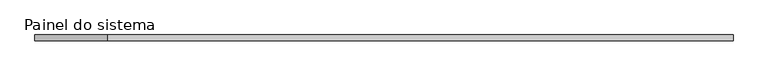
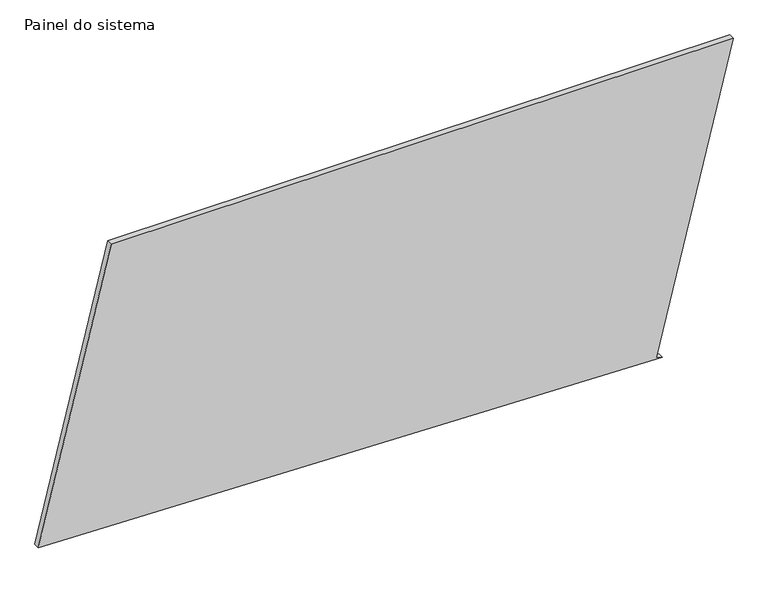
"""IFC4 building model written with IfcOpenShell, lengths in millimetres: plate geometry, Painel do sistema : Envidraçado."""

from ifc_helpers import new_model, si_unit, frame, origin, place, context, project, spatial, polyline, outline, extrude, source, transform, mapped, element, save


def painel_do_sistema_4682d0e1(model_context):
    return source(origin(), model_context, "Body", "SweptSolid", [
        extrude(outline(polyline([(0.0, 1166.435661), (5.9765403, 1142.160551), (1318.2584981, 1465.2448107), (1318.2584981, -1158.4600365), (72.1806963, -1465.2448107), (0.0, 1166.435661)])), frame((0.0, 24.5, 0.0), z_axis=(0.0, 1.0, 0.0), x_axis=(0.0, 0.0, 1.0)), (0.0, 0.0, 1.0), 25.0),
    ])


if __name__ == "__main__":
    model = new_model("IFC4")
    model_context = context("Model", 3, world=origin())
    ifc_project = project(units=[si_unit("LENGTHUNIT", "METRE", prefix="MILLI")], contexts=[model_context])
    site = spatial("IfcSite", under=ifc_project)
    building = spatial("IfcBuilding", under=site)
    placement = place(None, origin())
    painel_do_sistema_shape = painel_do_sistema_4682d0e1(model_context)
    element("IfcPlate", 1, ObjectType="Painel do sistema : Envidraçado", at=placement, inside=building, context=model_context, shape_type="MappedRepresentation", body=[
        mapped(painel_do_sistema_shape, transform((0.0, 0.0, 0.0), x_axis=(1.0, 0.0, 0.0), y_axis=(0.0, 1.0, 0.0), z_axis=(0.0, 0.0, 1.0))),
    ])
    save(model, "model.ifc")

# Revit data of these elements
# Type "Painel do sistema : Envidraçado"
#   Construction Type Id = "GSP4R"
#   Analytic Construction = "Vidraça única Pilkington 1/8 pol"
#   Visual Light Transmittance = 0.9
#   Solar Heat Gain Coefficient = 0.86
#   Heat Transfer Coefficient (U) = 6.7069 W/(m²·K)
# Element 1 (IfcPlate, "Painel do sistema : Envidraçado")
#   Materials on its faces: "Vidro"
# Materials
#   "Vidro": class "Vidro", colour RGB 0 128 192, transparency 0.9, Description = "Vidro de sílica", Cost = 0
